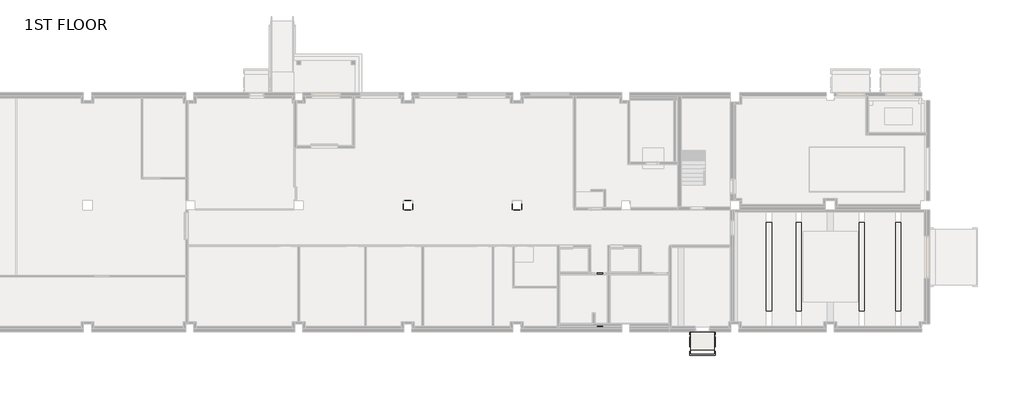
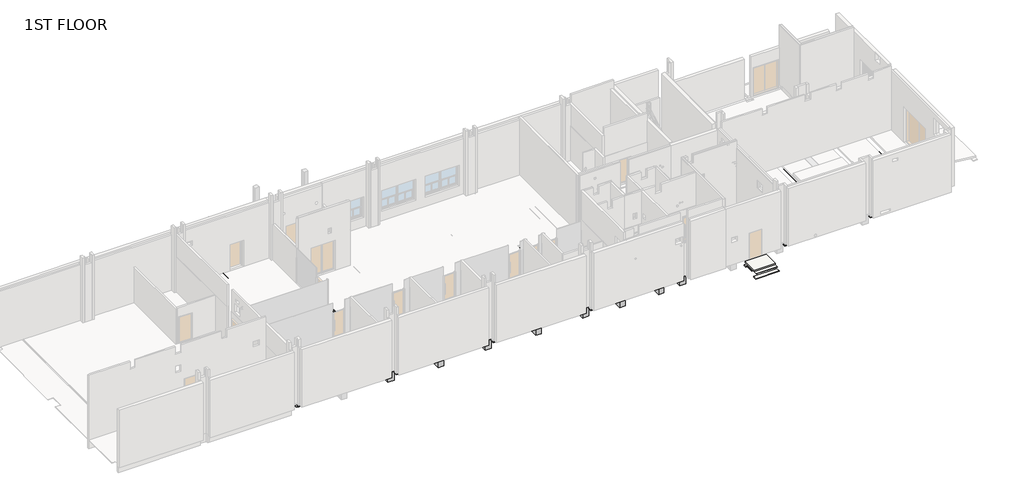
# One storey, part 9 of 15: 19 beams, 7 slabs.
"""IFC4 building model written with IfcOpenShell, lengths in millimetres."""

from ifc_helpers import new_model, si_unit, frame, origin, place, context, project, spatial, polyline, outline, extrude, faceted_brep, element, save

model = new_model("IFC4")

# Units and contexts
model_context = context("Model", 3, world=origin())
ifc_project = project(units=[si_unit("LENGTHUNIT", "METRE", prefix="MILLI")], contexts=[model_context])

# Site, building, storey
site = spatial("IfcSite", under=ifc_project)
building = spatial("IfcBuilding", under=site)
storey = spatial("IfcBuildingStorey", under=building, Name="1ST FLOOR", Elevation=4800.0)

# Beams
placement = place(None, origin())
element("IfcBeam", 1, ObjectType="RC Beam_Rectangular : H_SB_AR S16_TG-UG_500x800_1G2", at=placement, inside=storey, context=model_context, shape_type="Brep", body=[
    faceted_brep([(22650.0, -8350.0, 4800.0), (22650.0, -7850.0, 4800.0), (19225.0, -7850.0, 4800.0), (18775.0, -7850.0, 4800.0), (15400.0000001, -7850.0, 4800.0), (15400.0000001, -8350.0, 4800.0), (18775.0, -8350.0, 4800.0), (19225.0, -8350.0, 4800.0), (22650.0, -7850.0, 4000.0), (19225.0, -7850.0, 4000.0), (18775.0, -7850.0, 4000.0), (15400.0000001, -7850.0, 4000.0), (15400.0000001, -7850.0, 4650.0), (22650.0, -7850.0, 4650.0), (22650.0, -8350.0, 4000.0), (19225.0, -8350.0, 4000.0), (18775.0, -8350.0, 4000.0), (15400.0000001, -8350.0, 4000.0), (22650.0, -8350.0, 4650.0), (15400.0000001, -8350.0, 4650.0)], [[[0, 1, 2, 3, 4, 5, 6, 7]], [[8, 9, 10, 11, 12, 4, 3, 2, 1, 13]], [[11, 10, 9, 8, 14, 15, 16, 17]], [[17, 16, 15, 14, 18, 0, 7, 6, 5, 19]], [[14, 8, 13, 1, 0, 18]], [[5, 4, 12, 11, 17, 19]]]),
])
element("IfcBeam", 2, ObjectType="RC Beam_Rectangular : H_SB_AR S16_TG-UG_500x800_1G2", at=placement, inside=storey, context=model_context, shape_type="Brep", body=[
    faceted_brep([(23350.0, -7850.0, 4800.0), (23350.0, -8350.0, 4800.0), (26775.0, -8350.0, 4800.0), (27225.0, -8350.0, 4800.0), (30650.0, -8350.0, 4800.0), (30650.0, -7850.0, 4800.0), (27225.0, -7850.0, 4800.0), (26775.0, -7850.0, 4800.0), (23350.0, -8350.0, 4000.0), (26775.0, -8350.0, 4000.0), (27225.0, -8350.0, 4000.0), (30650.0, -8350.0, 4000.0), (30650.0, -8350.0, 4650.0), (23350.0, -8350.0, 4650.0), (23350.0, -7850.0, 4000.0), (26775.0, -7850.0, 4000.0), (27225.0, -7850.0, 4000.0), (30650.0, -7850.0, 4000.0), (23350.0, -7850.0, 4650.0), (30650.0, -7850.0, 4650.0)], [[[0, 1, 2, 3, 4, 5, 6, 7]], [[8, 9, 10, 11, 12, 4, 3, 2, 1, 13]], [[11, 10, 9, 8, 14, 15, 16, 17]], [[17, 16, 15, 14, 18, 0, 7, 6, 5, 19]], [[14, 8, 13, 1, 0, 18]], [[5, 4, 12, 11, 17, 19]]]),
])
element("IfcBeam", 3, ObjectType="RC Beam_Rectangular : H_SB_AR S16_TG-UG_500x800_1G2", at=placement, inside=storey, context=model_context, shape_type="Brep", body=[
    faceted_brep([(31350.0, -7850.0, 4800.0), (31350.0, -8350.0, 4800.0), (34775.0, -8350.0, 4800.0), (35225.0, -8350.0, 4800.0), (38650.0, -8350.0, 4800.0), (38650.0, -7850.0, 4800.0), (35225.0, -7850.0, 4800.0), (34775.0, -7850.0, 4800.0), (31350.0, -8350.0, 4000.0), (34775.0, -8350.0, 4000.0), (35225.0, -8350.0, 4000.0), (38650.0, -8350.0, 4000.0), (38650.0, -8350.0, 4650.0), (31350.0, -8350.0, 4650.0), (31350.0, -7850.0, 4000.0), (34775.0, -7850.0, 4000.0), (35225.0, -7850.0, 4000.0), (38650.0, -7850.0, 4000.0), (31350.0, -7850.0, 4650.0), (38650.0, -7850.0, 4650.0)], [[[0, 1, 2, 3, 4, 5, 6, 7]], [[8, 9, 10, 11, 12, 4, 3, 2, 1, 13]], [[11, 10, 9, 8, 14, 15, 16, 17]], [[17, 16, 15, 14, 18, 0, 7, 6, 5, 19]], [[14, 8, 13, 1, 0, 18]], [[5, 4, 12, 11, 17, 19]]]),
])
element("IfcBeam", 4, ObjectType="RC Beam_Rectangular : H_SB_AR S16_TG-UG_500x800_1G2", at=placement, inside=storey, context=model_context, shape_type="Brep", body=[
    faceted_brep([(39350.0, -7850.0, 4800.0), (39350.0, -8350.0, 4800.0), (41675.0, -8350.0, 4800.0), (42125.0, -8350.0, 4800.0), (44875.0, -8350.0, 4800.0), (45325.0, -8350.0, 4800.0), (46650.0, -8350.0, 4800.0), (46650.0, -7850.0, 4800.0), (45325.0, -7850.0, 4800.0), (44875.0, -7850.0, 4800.0), (42125.0, -7850.0, 4800.0), (41675.0, -7850.0, 4800.0), (39350.0, -8350.0, 4000.0), (41675.0, -8350.0, 4000.0), (42125.0, -8350.0, 4000.0), (44875.0, -8350.0, 4000.0), (45325.0, -8350.0, 4000.0), (46650.0, -8350.0, 4000.0), (46650.0, -8350.0, 4650.0), (39350.0, -8350.0, 4650.0), (39350.0, -7850.0, 4000.0), (41675.0, -7850.0, 4000.0), (42125.0, -7850.0, 4000.0), (44875.0, -7850.0, 4000.0), (45325.0, -7850.0, 4000.0), (46650.0, -7850.0, 4000.0), (39350.0, -7850.0, 4650.0), (46650.0, -7850.0, 4650.0)], [[[0, 1, 2, 3, 4, 5, 6, 7, 8, 9, 10, 11]], [[12, 13, 14, 15, 16, 17, 18, 6, 5, 4, 3, 2, 1, 19]], [[17, 16, 15, 14, 13, 12, 20, 21, 22, 23, 24, 25]], [[25, 24, 23, 22, 21, 20, 26, 0, 11, 10, 9, 8, 7, 27]], [[20, 12, 19, 1, 0, 26]], [[7, 6, 18, 17, 25, 27]]]),
])
element("IfcBeam", 5, ObjectType="RC Beam_Rectangular : H_SB_AR S16_TG-UG_500x800_1G1", at=placement, inside=storey, context=model_context, shape_type="Brep", body=[
    faceted_brep([(23200.0, -300.0, 4800.0), (22700.0, -300.0, 4800.0), (22700.0, -7650.0, 4800.0), (23200.0, -7650.0, 4800.0), (23200.0, -7650.0, 4650.0), (23200.0, -7650.0, 4000.0), (23200.0, -300.0, 4000.0), (23200.0, -300.0, 4650.0), (22700.0, -300.0, 4000.0), (22700.0, -7650.0, 4000.0), (22700.0, -300.0, 4650.0), (22700.0, -7650.0, 4650.0)], [[[0, 1, 2, 3]], [[0, 3, 4, 5, 6, 7]], [[8, 6, 5, 9]], [[2, 1, 10, 8, 9, 11]], [[1, 0, 7, 6, 8, 10]], [[3, 2, 11, 9, 5, 4]]]),
])
element("IfcBeam", 6, ObjectType="RC Beam_Rectangular : H_SB_AR S16_TG-UG_450x800_1B1", at=placement, inside=storey, context=model_context, shape_type="Brep", body=[
    faceted_brep([(19225.0, -100.0, 4800.0), (18775.0, -100.0, 4800.0), (18775.0, -7850.0, 4800.0), (19225.0, -7850.0, 4800.0), (19225.0, -7850.0, 4650.0), (19225.0, -7850.0, 4000.0), (19225.0, -100.0, 4000.0), (19225.0, -100.0, 4650.0), (18775.0, -100.0, 4000.0), (18775.0, -7850.0, 4000.0), (18775.0, -100.0, 4650.0), (18775.0, -7850.0, 4650.0)], [[[0, 1, 2, 3]], [[0, 3, 4, 5, 6, 7]], [[8, 6, 5, 9]], [[2, 1, 10, 8, 9, 11]], [[1, 0, 7, 6, 8, 10]], [[3, 2, 11, 9, 5, 4]]]),
])
element("IfcBeam", 7, ObjectType="RC Beam_Rectangular : H_SB_AR S16_TG-UG_500x800_1G1", at=placement, inside=storey, context=model_context, shape_type="Brep", body=[
    faceted_brep([(31250.0, -300.0, 4800.0), (30750.0, -300.0, 4800.0), (30750.0, -7650.0, 4800.0), (31250.0, -7650.0, 4800.0), (31250.0, -7650.0, 4650.0), (31250.0, -7650.0, 4000.0), (31250.0, -300.0, 4000.0), (31250.0, -300.0, 4650.0), (30750.0, -300.0, 4000.0), (30750.0, -7650.0, 4000.0), (30750.0, -300.0, 4650.0), (30750.0, -7650.0, 4650.0)], [[[0, 1, 2, 3]], [[0, 3, 4, 5, 6, 7]], [[8, 6, 5, 9]], [[2, 1, 10, 8, 9, 11]], [[1, 0, 7, 6, 8, 10]], [[3, 2, 11, 9, 5, 4]]]),
])
element("IfcBeam", 8, ObjectType="RC Beam_Rectangular : H_SB_AR S16_TG-UG_450x800_1B1", at=placement, inside=storey, context=model_context, shape_type="Brep", body=[
    faceted_brep([(27225.0, -100.0, 4800.0), (26775.0, -100.0, 4800.0), (26775.0, -7850.0, 4800.0), (27225.0, -7850.0, 4800.0), (27225.0, -7850.0, 4650.0), (27225.0, -7850.0, 4000.0), (27225.0, -100.0, 4000.0), (27225.0, -100.0, 4650.0), (26775.0, -100.0, 4000.0), (26775.0, -7850.0, 4000.0), (26775.0, -100.0, 4650.0), (26775.0, -7850.0, 4650.0)], [[[0, 1, 2, 3]], [[0, 3, 4, 5, 6, 7]], [[8, 6, 5, 9]], [[2, 1, 10, 8, 9, 11]], [[1, 0, 7, 6, 8, 10]], [[3, 2, 11, 9, 5, 4]]]),
])
element("IfcBeam", 9, ObjectType="RC Beam_Rectangular : H_SB_AR S16_TG-UG_450x800_1B1", at=placement, inside=storey, context=model_context, shape_type="Brep", body=[
    faceted_brep([(35225.0, -100.0, 4800.0), (34775.0, -100.0, 4800.0), (34775.0, -7850.0, 4800.0), (35225.0, -7850.0, 4800.0), (35225.0, -7850.0, 4650.0), (35225.0, -7850.0, 4000.0), (35225.0, -100.0, 4000.0), (35225.0, -100.0, 4650.0), (34775.0, -100.0, 4000.0), (34775.0, -7850.0, 4000.0), (34775.0, -100.0, 4650.0), (34775.0, -7850.0, 4650.0)], [[[0, 1, 2, 3]], [[0, 3, 4, 5, 6, 7]], [[8, 6, 5, 9]], [[2, 1, 10, 8, 9, 11]], [[1, 0, 7, 6, 8, 10]], [[3, 2, 11, 9, 5, 4]]]),
])
element("IfcBeam", 10, ObjectType="RC Beam_Rectangular : H_SB_AR S16_TG-UG_500x800_1G1", at=placement, inside=storey, context=model_context, shape_type="Brep", body=[
    faceted_brep([(22750.0, -16700.0, 4800.0), (23250.0, -16700.0, 4800.0), (23250.0, -8350.0, 4800.0), (22750.0, -8350.0, 4800.0), (23250.0, -16700.0, 4650.0), (23250.0, -16700.0, 4000.0), (23250.0, -8350.0, 4000.0), (23250.0, -8350.0, 4650.0), (22750.0, -16700.0, 4000.0), (22750.0, -8350.0, 4000.0), (22750.0, -16700.0, 4650.0), (22750.0, -8350.0, 4650.0)], [[[0, 1, 2, 3]], [[1, 4, 5, 6, 7, 2]], [[5, 8, 9, 6]], [[8, 10, 0, 3, 11, 9]], [[8, 5, 4, 1, 0, 10]], [[3, 2, 7, 6, 9, 11]]]),
])
element("IfcBeam", 11, ObjectType="RC Beam_Rectangular : H_SB_AR S16_TG-UG_500x800_1G1", at=placement, inside=storey, context=model_context, shape_type="Brep", body=[
    faceted_brep([(30750.0, -16700.0, 4800.0), (31250.0, -16700.0, 4800.0), (31250.0, -8350.0, 4800.0), (30750.0, -8350.0, 4800.0), (31250.0, -16700.0, 4650.0), (31250.0, -16700.0, 4000.0), (31250.0, -8350.0, 4000.0), (31250.0, -8350.0, 4650.0), (30750.0, -16700.0, 4000.0), (30750.0, -8350.0, 4000.0), (30750.0, -16700.0, 4650.0), (30750.0, -8350.0, 4650.0)], [[[0, 1, 2, 3]], [[1, 4, 5, 6, 7, 2]], [[5, 8, 9, 6]], [[8, 10, 0, 3, 11, 9]], [[8, 5, 4, 1, 0, 10]], [[3, 2, 7, 6, 9, 11]]]),
])
element("IfcBeam", 12, ObjectType="RC Beam_Rectangular : H_SB_AR S16_TG-UG_500x800_1G1", at=placement, inside=storey, context=model_context, shape_type="Brep", body=[
    faceted_brep([(38750.0000001, -16700.0, 4800.0), (39250.0000001, -16700.0, 4800.0), (39250.0000001, -8350.0, 4800.0), (38750.0000001, -8350.0, 4800.0), (39250.0000001, -16700.0, 4650.0), (39250.0000001, -16700.0, 4000.0), (39250.0000001, -8350.0, 4000.0), (39250.0000001, -8350.0, 4650.0), (38750.0000001, -16700.0, 4000.0), (38750.0000001, -8350.0, 4000.0), (38750.0000001, -16700.0, 4650.0), (38750.0000001, -8350.0, 4650.0)], [[[0, 1, 2, 3]], [[1, 4, 5, 6, 7, 2]], [[5, 8, 9, 6]], [[8, 10, 0, 3, 11, 9]], [[8, 5, 4, 1, 0, 10]], [[3, 2, 7, 6, 9, 11]]]),
])
element("IfcBeam", 13, ObjectType="RC Beam_Rectangular : H_SB_AR S16_TG-UG_450x800_1B1A", at=placement, inside=storey, context=model_context, shape_type="Brep", body=[
    faceted_brep([(26775.0, -16900.0, 4800.0), (27225.0, -16900.0, 4800.0), (27225.0, -8350.0, 4800.0), (26775.0, -8350.0, 4800.0), (27225.0, -16900.0, 4650.0), (27225.0, -16900.0, 4000.0), (27225.0, -8350.0, 4000.0), (27225.0, -8350.0, 4650.0), (26775.0, -16900.0, 4000.0), (26775.0, -8350.0, 4000.0), (26775.0, -8350.0, 4650.0), (26775.0, -16900.0, 4650.0)], [[[0, 1, 2, 3]], [[2, 1, 4, 5, 6, 7]], [[5, 8, 9, 6]], [[0, 3, 10, 9, 8, 11]], [[1, 0, 11, 8, 5, 4]], [[3, 2, 7, 6, 9, 10]]]),
])
element("IfcBeam", 14, ObjectType="RC Beam_Rectangular : H_SB_AR S16_TG-UG_450x800_1B1A", at=placement, inside=storey, context=model_context, shape_type="Brep", body=[
    faceted_brep([(34775.0, -16900.0, 4800.0), (35225.0, -16900.0, 4800.0), (35225.0, -8350.0, 4800.0), (34775.0, -8350.0, 4800.0), (35225.0, -16900.0, 4650.0), (35225.0, -16900.0, 4000.0), (35225.0, -8350.0, 4000.0), (35225.0, -8350.0, 4650.0), (34775.0, -16900.0, 4000.0), (34775.0, -8350.0, 4000.0), (34775.0, -8350.0, 4650.0), (34775.0, -16900.0, 4650.0)], [[[0, 1, 2, 3]], [[2, 1, 4, 5, 6, 7]], [[5, 8, 9, 6]], [[0, 3, 10, 9, 8, 11]], [[1, 0, 11, 8, 5, 4]], [[3, 2, 7, 6, 9, 10]]]),
])
element("IfcBeam", 15, ObjectType="RC Beam_Rectangular : H_SB_AR S16_TG-UG_450x800_1B1A", at=placement, inside=storey, context=model_context, shape_type="Brep", body=[
    faceted_brep([(42125.0, -8350.0, 4800.0), (41675.0, -8350.0, 4800.0), (41675.0, -16900.0, 4800.0), (42125.0, -16900.0, 4800.0), (42125.0, -11075.0, 4800.0), (42125.0, -16900.0, 4700.0), (42125.0, -16900.0, 4550.0), (42125.0, -16900.0, 4000.0), (42125.0, -8350.0, 4000.0), (42125.0, -8350.0, 4650.0), (41675.0, -16900.0, 4000.0), (41675.0, -8350.0, 4000.0), (41675.0, -16900.0, 4650.0), (41675.0, -8350.0, 4650.0)], [[[0, 1, 2, 3, 4]], [[3, 5, 6, 7, 8, 9, 0, 4]], [[7, 10, 11, 8]], [[11, 10, 12, 2, 1, 13]], [[7, 6, 5, 3, 2, 12, 10]], [[1, 0, 9, 8, 11, 13]]]),
])
element("IfcBeam", 16, ObjectType="RC Beam_Rectangular : H_SB_AR S16_TG-UG_450x700_1B1B", at=placement, inside=storey, context=model_context, shape_type="Brep", body=[
    faceted_brep([(44875.0, -13075.0, 4700.0), (45325.0, -13075.0, 4700.0), (45325.0, -13075.0, 4650.0), (45325.0, -13075.0, 4550.0), (45325.0, -13075.0, 4000.0), (44875.0, -13075.0, 4000.0), (44875.0, -13075.0, 4550.0), (44875.0, -13075.0, 4650.0), (44875.0, -16900.0, 4700.0), (45325.0, -16900.0, 4700.0), (45325.0, -16900.0, 4550.0), (45325.0, -16900.0, 4000.0), (44875.0, -16900.0, 4000.0), (44875.0, -16900.0, 4550.0)], [[[0, 1, 2, 3, 4, 5, 6, 7]], [[1, 0, 8, 9]], [[1, 9, 10, 11, 4, 3, 2]], [[5, 4, 11, 12]], [[8, 0, 7, 6, 5, 12, 13]], [[12, 11, 10, 9, 8, 13]]]),
])
element("IfcBeam", 17, ObjectType="RC Beam_Rectangular : H_SB_AR S16_TG-UG_500x700_1G1A", at=placement, inside=storey, context=model_context, shape_type="Brep", body=[
    faceted_brep([(46750.0, -11075.0, 4700.0), (47250.0, -11075.0, 4700.0), (47250.0, -11075.0, 4550.0), (47250.0, -11075.0, 4000.0), (46750.0, -11075.0, 4000.0), (46750.0, -11075.0, 4550.0), (46750.0, -16700.0, 4700.0), (47250.0, -16700.0, 4700.0), (47250.0, -16700.0, 4550.0), (47250.0, -16700.0, 4000.0), (46750.0, -16700.0, 4000.0), (46750.0, -16700.0, 4550.0)], [[[0, 1, 2, 3, 4, 5]], [[1, 0, 6, 7]], [[1, 7, 8, 9, 3, 2]], [[4, 3, 9, 10]], [[6, 0, 5, 4, 10, 11]], [[10, 9, 8, 7, 6, 11]]]),
])
element("IfcBeam", 18, ObjectType="RC Beam_Rectangular : H_SB_AR S16_TG-UG_500x800_1G1A", at=placement, inside=storey, context=model_context, shape_type="Brep", body=[
    faceted_brep([(46750.0, -11075.0, 4000.0), (47250.0, -11075.0, 4000.0), (47250.0, -11075.0, 4650.0), (47250.0, -11075.0, 4700.0), (47250.0, -11075.0, 4800.0), (46750.0, -11075.0, 4800.0), (46750.0, -11075.0, 4700.0), (46750.0, -11075.0, 4650.0), (47249.9999999, -8350.0, 4800.0), (46749.9999999, -8350.0, 4800.0), (47249.9999999, -8350.0, 4000.0), (47249.9999999, -8350.0, 4650.0), (46749.9999999, -8350.0, 4000.0), (46749.9999999, -8350.0, 4650.0)], [[[0, 1, 2, 3, 4, 5, 6, 7]], [[5, 4, 8, 9]], [[2, 1, 10, 11, 8, 4, 3]], [[1, 0, 12, 10]], [[7, 6, 5, 9, 13, 12, 0]], [[9, 8, 11, 10, 12, 13]]]),
])
element("IfcBeam", 19, ObjectType="RC Beam_Rectangular : H_SB_AR S16_TG-UG_450x800_1B1B", at=placement, inside=storey, context=model_context, shape_type="Brep", body=[
    faceted_brep([(44875.0, -13075.0, 4000.0), (45325.0, -13075.0, 4000.0), (45325.0, -13075.0, 4650.0), (45325.0, -13075.0, 4700.0), (45325.0, -13075.0, 4800.0), (44875.0, -13075.0, 4800.0), (44875.0, -13075.0, 4700.0), (44875.0, -13075.0, 4650.0), (45325.0, -8350.0, 4800.0), (44875.0, -8350.0, 4800.0), (45325.0, -8350.0, 4000.0), (45325.0, -8350.0, 4650.0), (44875.0, -8350.0, 4000.0), (44875.0, -8350.0, 4650.0)], [[[0, 1, 2, 3, 4, 5, 6, 7]], [[5, 4, 8, 9]], [[8, 4, 3, 2, 1, 10, 11]], [[1, 0, 12, 10]], [[5, 9, 13, 12, 0, 7, 6]], [[9, 8, 11, 10, 12, 13]]]),
])

# Slabs
element("IfcSlab", 20, ObjectType="H_SF_AR_B08_Stoop_T150", at=placement, inside=storey, context=model_context, shape_type="Brep", body=[
    faceted_brep([(51775.0, -18599.9999926, 4600.0), (51775.0, -18399.9999926, 4600.0), (51775.0, -17662.0, 4600.0), (51775.0, -17312.0, 4600.0), (53475.0, -17312.0, 4600.0), (53475.0, -17662.0, 4600.0), (53475.0, -18399.9999926, 4600.0), (53475.0, -18599.9999926, 4600.0), (51775.0, -18599.9999926, 4750.0), (53475.0, -18599.9999926, 4750.0), (53475.0, -17312.0, 4750.0), (51775.0, -17312.0, 4750.0), (51775.0, -18599.9999926, 4625.0), (53475.0, -18599.9999926, 4625.0)], [[[0, 1, 2, 3, 4, 5, 6, 7]], [[8, 9, 10, 11]], [[3, 2, 1, 0, 12, 8, 11]], [[4, 3, 11, 10]], [[7, 6, 5, 4, 10, 9, 13]], [[0, 7, 13, 9, 8, 12]]]),
])
element("IfcSlab", 21, ObjectType="H_SF_AR_B08_Stoop_T125", at=placement, inside=storey, context=model_context, shape_type="SweptSolid", body=[
    extrude(outline(polyline([(51775.0, -18899.9999926), (51775.0, -18599.9999926), (53475.0, -18599.9999926), (53475.0, -18899.9999926), (51775.0, -18899.9999926)])), frame((0.0, 0.0, 4600.0), z_axis=(0.0, 0.0, 1.0), x_axis=(1.0, 0.0, 0.0)), (0.0, 0.0, 1.0), 25.0),
])
element("IfcSlab", 22, ObjectType="H_SF_AR_S18_Lean_T50", at=placement, inside=storey, context=model_context, shape_type="SweptSolid", body=[
    extrude(outline(polyline([(51675.0, -18999.9999926), (51675.0, -18699.9999926), (53575.0, -18699.9999926), (53575.0, -18999.9999926), (51675.0, -18999.9999926)])), frame((0.0, 0.0, 4250.0), z_axis=(0.0, 0.0, 1.0), x_axis=(1.0, 0.0, 0.0)), (0.0, 0.0, 1.0), 50.0),
])
element("IfcSlab", 23, ObjectType="H_SF_AR_S18_Lean_T50", at=placement, inside=storey, context=model_context, shape_type="SweptSolid", body=[
    extrude(outline(polyline([(51675.0, -17299.9999926), (53575.0, -17299.9999926), (53575.0, -17512.0), (51675.0, -17512.0), (51675.0, -17299.9999926)])), frame((0.0, 0.0, 4400.0), z_axis=(0.0, 0.0, 1.0), x_axis=(1.0, 0.0, 0.0)), (0.0, 0.0, 1.0), 50.0),
])
element("IfcSlab", 24, ObjectType="H_SF_AR_S18_Lean_T50", at=placement, inside=storey, context=model_context, shape_type="Brep", body=[
    faceted_brep([(51675.0, -18399.9999926, 4550.0), (51675.0, -18379.2893145, 4550.0), (51675.0, -17682.7106781, 4550.0), (51675.0, -17662.0, 4550.0), (53575.0, -17662.0, 4550.0), (53575.0, -17682.7106781, 4550.0), (53575.0, -18379.2893145, 4550.0), (53575.0, -18399.9999926, 4550.0), (51675.0, -18399.9999926, 4600.0), (53575.0, -18399.9999926, 4600.0), (53575.0, -17662.0, 4600.0), (51675.0, -17662.0, 4600.0)], [[[0, 1, 2, 3, 4, 5, 6, 7]], [[8, 9, 10, 11]], [[3, 2, 1, 0, 8, 11]], [[4, 3, 11, 10]], [[7, 6, 5, 4, 10, 9]], [[0, 7, 9, 8]]]),
])
element("IfcSlab", 25, ObjectType="H_SF_AR_S18_Lean_T50", at=placement, inside=storey, context=model_context, shape_type="Brep", body=[
    faceted_brep([(19435.0, -1250.0000001, 3840.0), (19435.0, -7640.0, 3840.0), (21750.0000003, -7640.0, 3840.0), (21750.0000003, -8560.0, 3840.0), (19435.0, -8560.0, 3840.0), (19435.0, -15750.0000001, 3840.0), (18565.0, -15750.0000001, 3840.0), (18565.0, -8560.0, 3840.0), (16300.0000001, -8560.0, 3840.0), (16300.0000001, -7640.0, 3840.0), (18565.0, -7640.0, 3840.0), (18565.0, -1250.0000001, 3840.0), (19435.0, -7640.0, 3890.0), (19435.0, -1250.0000001, 3890.0), (18565.0, -1250.0000001, 3890.0), (18565.0, -7640.0, 3890.0), (16300.0000001, -7640.0, 3890.0), (16300.0000001, -8560.0, 3890.0), (18565.0, -8560.0, 3890.0), (18565.0, -15750.0000001, 3890.0), (19435.0, -15750.0000001, 3890.0), (19435.0, -8560.0, 3890.0), (21750.0000003, -8560.0, 3890.0), (21750.0000003, -7640.0, 3890.0)], [[[0, 1, 2, 3, 4, 5, 6, 7, 8, 9, 10, 11]], [[12, 13, 14, 15, 16, 17, 18, 19, 20, 21, 22, 23]], [[1, 0, 13, 12]], [[2, 1, 12, 23]], [[3, 2, 23, 22]], [[4, 3, 22, 21]], [[5, 4, 21, 20]], [[7, 6, 19, 18]], [[8, 7, 18, 17]], [[9, 8, 17, 16]], [[10, 9, 16, 15]], [[11, 10, 15, 14]], [[0, 11, 14, 13]], [[6, 5, 20, 19]]]),
    faceted_brep([(23410.0, -1250.0000001, 3840.0), (23410.0, -6750.0, 3840.0), (22490.0, -6750.0, 3840.0), (22490.0, -1250.0000001, 3840.0), (23410.0, -6750.0, 3890.0), (23410.0, -1250.0000001, 3890.0), (22490.0, -1250.0000001, 3890.0), (22490.0, -6750.0, 3890.0)], [[[0, 1, 2, 3]], [[4, 5, 6, 7]], [[1, 0, 5, 4]], [[2, 1, 4, 7]], [[3, 2, 7, 6]], [[0, 3, 6, 5]]]),
    faceted_brep([(23460.0, -9250.0, 3840.0), (23460.0, -15750.0000001, 3840.0), (22540.0, -15750.0000001, 3840.0), (22540.0, -9250.0, 3840.0), (23460.0, -15750.0000001, 3890.0), (23460.0, -9250.0, 3890.0), (22540.0, -9250.0, 3890.0), (22540.0, -15750.0000001, 3890.0)], [[[0, 1, 2, 3]], [[4, 5, 6, 7]], [[1, 0, 5, 4]], [[2, 1, 4, 7]], [[3, 2, 7, 6]], [[0, 3, 6, 5]]]),
    faceted_brep([(27435.0, -1250.0000001, 3840.0), (27435.0, -7640.0, 3840.0), (29750.0000003, -7640.0, 3840.0), (29750.0000003, -8560.0, 3840.0), (27435.0, -8560.0, 3840.0), (27435.0, -15750.0000001, 3840.0), (26565.0, -15750.0000001, 3840.0), (26565.0, -8560.0, 3840.0), (24249.9999997, -8560.0, 3840.0), (24249.9999997, -7640.0, 3840.0), (26565.0, -7640.0, 3840.0), (26565.0, -1250.0000001, 3840.0), (27435.0, -7640.0, 3890.0), (27435.0, -1250.0000001, 3890.0), (26565.0, -1250.0000001, 3890.0), (26565.0, -7640.0, 3890.0), (24249.9999997, -7640.0, 3890.0), (24249.9999997, -8560.0, 3890.0), (26565.0, -8560.0, 3890.0), (26565.0, -15750.0000001, 3890.0), (27435.0, -15750.0000001, 3890.0), (27435.0, -8560.0, 3890.0), (29750.0000003, -8560.0, 3890.0), (29750.0000003, -7640.0, 3890.0)], [[[0, 1, 2, 3, 4, 5, 6, 7, 8, 9, 10, 11]], [[12, 13, 14, 15, 16, 17, 18, 19, 20, 21, 22, 23]], [[1, 0, 13, 12]], [[2, 1, 12, 23]], [[3, 2, 23, 22]], [[4, 3, 22, 21]], [[5, 4, 21, 20]], [[6, 5, 20, 19]], [[7, 6, 19, 18]], [[8, 7, 18, 17]], [[9, 8, 17, 16]], [[10, 9, 16, 15]], [[11, 10, 15, 14]], [[0, 11, 14, 13]]]),
    faceted_brep([(31459.9999999, -1250.0000001, 3840.0), (31459.9999999, -6750.0, 3840.0), (30539.9999999, -6750.0, 3840.0), (30539.9999999, -1250.0000001, 3840.0), (31459.9999999, -6750.0, 3890.0), (31459.9999999, -1250.0000001, 3890.0), (30539.9999999, -1250.0000001, 3890.0), (30539.9999999, -6750.0, 3890.0)], [[[0, 1, 2, 3]], [[4, 5, 6, 7]], [[1, 0, 5, 4]], [[2, 1, 4, 7]], [[3, 2, 7, 6]], [[0, 3, 6, 5]]]),
    faceted_brep([(31459.9999999, -9250.0, 3840.0), (31459.9999999, -15750.0000001, 3840.0), (30539.9999999, -15750.0000001, 3840.0), (30539.9999999, -9250.0, 3840.0), (31459.9999999, -15750.0000001, 3890.0), (31459.9999999, -9250.0, 3890.0), (30539.9999999, -9250.0, 3890.0), (30539.9999999, -15750.0000001, 3890.0)], [[[0, 1, 2, 3]], [[4, 5, 6, 7]], [[1, 0, 5, 4]], [[2, 1, 4, 7]], [[3, 2, 7, 6]], [[0, 3, 6, 5]]]),
    faceted_brep([(35435.0, -1250.0000001, 3840.0), (35435.0, -7640.0, 3840.0), (37750.0000003, -7640.0, 3840.0), (37750.0000003, -8560.0, 3840.0), (35435.0, -8560.0, 3840.0), (35435.0, -15750.0000001, 3840.0), (34565.0, -15750.0000001, 3840.0), (34565.0, -8560.0, 3840.0), (32250.0000002, -8560.0, 3840.0), (32250.0000002, -7640.0, 3840.0), (34565.0, -7640.0, 3840.0), (34565.0, -1250.0000001, 3840.0), (35435.0, -7640.0, 3890.0), (35435.0, -1250.0000001, 3890.0), (34565.0, -1250.0000001, 3890.0), (34565.0, -7640.0, 3890.0), (32250.0000002, -7640.0, 3890.0), (32250.0000002, -8560.0, 3890.0), (34565.0, -8560.0, 3890.0), (34565.0, -15750.0000001, 3890.0), (35435.0, -15750.0000001, 3890.0), (35435.0, -8560.0, 3890.0), (37750.0000003, -8560.0, 3890.0), (37750.0000003, -7640.0, 3890.0)], [[[0, 1, 2, 3, 4, 5, 6, 7, 8, 9, 10, 11]], [[12, 13, 14, 15, 16, 17, 18, 19, 20, 21, 22, 23]], [[1, 0, 13, 12]], [[2, 1, 12, 23]], [[3, 2, 23, 22]], [[4, 3, 22, 21]], [[5, 4, 21, 20]], [[6, 5, 20, 19]], [[7, 6, 19, 18]], [[8, 7, 18, 17]], [[9, 8, 17, 16]], [[10, 9, 16, 15]], [[11, 10, 15, 14]], [[0, 11, 14, 13]]]),
    faceted_brep([(39459.9999999, -1250.0000001, 3840.0), (39459.9999999, -6750.0, 3840.0), (38539.9999999, -6750.0, 3840.0), (38539.9999999, -1250.0000001, 3840.0), (39459.9999999, -6750.0, 3890.0), (39459.9999999, -1250.0000001, 3890.0), (38539.9999999, -1250.0000001, 3890.0), (38539.9999999, -6750.0, 3890.0)], [[[0, 1, 2, 3]], [[4, 5, 6, 7]], [[1, 0, 5, 4]], [[2, 1, 4, 7]], [[3, 2, 7, 6]], [[0, 3, 6, 5]]]),
    faceted_brep([(39459.9999999, -9250.0, 3840.0), (39459.9999999, -15750.0000001, 3840.0), (38539.9999999, -15750.0000001, 3840.0), (38539.9999999, -9250.0, 3840.0), (39459.9999999, -15750.0000001, 3890.0), (39459.9999999, -9250.0, 3890.0), (38539.9999999, -9250.0, 3890.0), (38539.9999999, -15750.0000001, 3890.0)], [[[0, 1, 2, 3]], [[4, 5, 6, 7]], [[1, 0, 5, 4]], [[2, 1, 4, 7]], [[3, 2, 7, 6]], [[0, 3, 6, 5]]]),
    faceted_brep([(42335.0, -1250.0000001, 3840.0), (42335.0, -7640.0, 3840.0), (44665.0, -7640.0, 3840.0), (44665.0, -1250.0000001, 3840.0), (45535.0, -1250.0000001, 3840.0), (45535.0, -7640.0, 3840.0), (45749.9999999, -7640.0, 3840.0), (45749.9999999, -8560.0, 3840.0), (45535.0, -8560.0, 3840.0), (45535.0, -15750.0000001, 3840.0), (44665.0, -15750.0000001, 3840.0), (44665.0, -8560.0, 3840.0), (42335.0, -8560.0, 3840.0), (42335.0, -15750.0000001, 3840.0), (41465.0, -15750.0000001, 3840.0), (41465.0, -8560.0, 3840.0), (40250.0000001, -8560.0, 3840.0), (40250.0000001, -7640.0, 3840.0), (41465.0, -7640.0, 3840.0), (41465.0, -1250.0000001, 3840.0), (42335.0, -7640.0, 3890.0), (42335.0, -1250.0000001, 3890.0), (41465.0, -1250.0000001, 3890.0), (41465.0, -7640.0, 3890.0), (40250.0000001, -7640.0, 3890.0), (40250.0000001, -8560.0, 3890.0), (41465.0, -8560.0, 3890.0), (41465.0, -15750.0000001, 3890.0), (42335.0, -15750.0000001, 3890.0), (42335.0, -8560.0, 3890.0), (44665.0, -8560.0, 3890.0), (44665.0, -15750.0000001, 3890.0), (45535.0, -15750.0000001, 3890.0), (45535.0, -8560.0, 3890.0), (45749.9999999, -8560.0, 3890.0), (45749.9999999, -7640.0, 3890.0), (45535.0, -7640.0, 3890.0), (45535.0, -1250.0000001, 3890.0), (44665.0, -1250.0000001, 3890.0), (44665.0, -7640.0, 3890.0)], [[[0, 1, 2, 3, 4, 5, 6, 7, 8, 9, 10, 11, 12, 13, 14, 15, 16, 17, 18, 19]], [[20, 21, 22, 23, 24, 25, 26, 27, 28, 29, 30, 31, 32, 33, 34, 35, 36, 37, 38, 39]], [[1, 0, 21, 20]], [[2, 1, 20, 39]], [[3, 2, 39, 38]], [[4, 3, 38, 37]], [[5, 4, 37, 36]], [[6, 5, 36, 35]], [[7, 6, 35, 34]], [[8, 7, 34, 33]], [[9, 8, 33, 32]], [[10, 9, 32, 31]], [[11, 10, 31, 30]], [[12, 11, 30, 29]], [[13, 12, 29, 28]], [[14, 13, 28, 27]], [[15, 14, 27, 26]], [[16, 15, 26, 25]], [[17, 16, 25, 24]], [[18, 17, 24, 23]], [[19, 18, 23, 22]], [[0, 19, 22, 21]]]),
    faceted_brep([(47509.9999996, -1250.0000001, 3840.0), (47509.9999996, -6750.0, 3840.0), (46589.9999996, -6750.0, 3840.0), (46589.9999996, -1250.0000001, 3840.0), (47509.9999996, -6750.0, 3890.0), (47509.9999996, -1250.0000001, 3890.0), (46589.9999996, -1250.0000001, 3890.0), (46589.9999996, -6750.0, 3890.0)], [[[0, 1, 2, 3]], [[4, 5, 6, 7]], [[1, 0, 5, 4]], [[2, 1, 4, 7]], [[3, 2, 7, 6]], [[0, 3, 6, 5]]]),
    faceted_brep([(47459.9999996, -9250.0, 3840.0), (47459.9999996, -15750.0000001, 3840.0), (47300.0, -15750.0000001, 3840.0), (46539.9999996, -15750.0000001, 3840.0), (46539.9999996, -9250.0, 3840.0), (47459.9999996, -15750.0000001, 3890.0), (47459.9999996, -9250.0, 3890.0), (46539.9999996, -9250.0, 3890.0), (46539.9999996, -15750.0000001, 3890.0), (47300.0, -15750.0000001, 3890.0)], [[[0, 1, 2, 3, 4]], [[5, 6, 7, 8, 9]], [[1, 0, 6, 5]], [[1, 5, 9, 8, 3, 2]], [[4, 3, 8, 7]], [[0, 4, 7, 6]]]),
    faceted_brep([(49700.0000002, -8560.0, 3840.0), (48249.9999999, -8560.0, 3840.0), (48249.9999999, -7640.0, 3840.0), (49700.0000002, -7640.0, 3840.0), (48249.9999999, -8560.0, 3890.0), (49700.0000002, -8560.0, 3890.0), (49700.0000002, -7640.0, 3890.0), (48249.9999999, -7640.0, 3890.0)], [[[0, 1, 2, 3]], [[4, 5, 6, 7]], [[1, 0, 5, 4]], [[2, 1, 4, 7]], [[3, 2, 7, 6]], [[0, 3, 6, 5]]]),
    faceted_brep([(50615.0, -15750.0000001, 3840.0), (50615.0, -9250.0, 3840.0), (51485.0, -9250.0, 3840.0), (51485.0, -15750.0000001, 3840.0), (50825.0, -15750.0000001, 3840.0), (50615.0, -9250.0, 3890.0), (50615.0, -15750.0000001, 3890.0), (50825.0, -15750.0000001, 3890.0), (51485.0, -15750.0000001, 3890.0), (51485.0, -9250.0, 3890.0)], [[[0, 1, 2, 3, 4]], [[5, 6, 7, 8, 9]], [[1, 0, 6, 5]], [[2, 1, 5, 9]], [[3, 2, 9, 8]], [[3, 8, 7, 6, 0, 4]]]),
    faceted_brep([(54490.0, -15750.0000001, 3840.0), (54490.0, -9250.0, 3840.0), (55410.0, -9250.0, 3840.0), (55410.0, -15750.0000001, 3840.0), (54490.0, -9250.0, 3890.0), (54490.0, -15750.0000001, 3890.0), (55410.0, -15750.0000001, 3890.0), (55410.0, -9250.0, 3890.0)], [[[0, 1, 2, 3]], [[4, 5, 6, 7]], [[1, 0, 5, 4]], [[2, 1, 4, 7]], [[3, 2, 7, 6]], [[0, 3, 6, 5]]]),
    faceted_brep([(57065.0, -15750.0000001, 3840.0), (57065.0, -9250.0, 3840.0), (57935.0, -9250.0, 3840.0), (57935.0, -15750.0000001, 3840.0), (57065.0, -9250.0, 3890.0), (57065.0, -15750.0000001, 3890.0), (57935.0, -15750.0000001, 3890.0), (57935.0, -9250.0, 3890.0)], [[[0, 1, 2, 3]], [[4, 5, 6, 7]], [[1, 0, 5, 4]], [[2, 1, 4, 7]], [[3, 2, 7, 6]], [[0, 3, 6, 5]]]),
    faceted_brep([(59265.0, -15750.0000001, 3840.0), (59265.0, -9250.0, 3840.0), (60135.0, -9250.0, 3840.0), (60135.0, -15750.0000001, 3840.0), (59265.0, -9250.0, 3890.0), (59265.0, -15750.0000001, 3890.0), (60135.0, -15750.0000001, 3890.0), (60135.0, -9250.0, 3890.0)], [[[0, 1, 2, 3]], [[4, 5, 6, 7]], [[1, 0, 5, 4]], [[2, 1, 4, 7]], [[3, 2, 7, 6]], [[0, 3, 6, 5]]]),
    faceted_brep([(61540.0, -15750.0000001, 3840.0), (61540.0, -9250.0, 3840.0), (62460.0, -9250.0, 3840.0), (62460.0, -15750.0000001, 3840.0), (61540.0, -9250.0, 3890.0), (61540.0, -15750.0000001, 3890.0), (62460.0, -15750.0000001, 3890.0), (62460.0, -9250.0, 3890.0)], [[[0, 1, 2, 3]], [[4, 5, 6, 7]], [[1, 0, 5, 4]], [[2, 1, 4, 7]], [[3, 2, 7, 6]], [[0, 3, 6, 5]]]),
    faceted_brep([(63865.0, -15750.0000001, 3840.0), (63865.0, -9250.0, 3840.0), (64735.0, -9250.0, 3840.0), (64735.0, -15750.0000001, 3840.0), (63865.0, -9250.0, 3890.0), (63865.0, -15750.0000001, 3890.0), (64735.0, -15750.0000001, 3890.0), (64735.0, -9250.0, 3890.0)], [[[0, 1, 2, 3]], [[4, 5, 6, 7]], [[1, 0, 5, 4]], [[2, 1, 4, 7]], [[3, 2, 7, 6]], [[0, 3, 6, 5]]]),
    faceted_brep([(66565.0, -15750.0000001, 3840.0), (66565.0, -9250.0, 3840.0), (67435.0, -9250.0, 3840.0), (67435.0, -15750.0000001, 3840.0), (66565.0, -9250.0, 3890.0), (66565.0, -15750.0000001, 3890.0), (67435.0, -15750.0000001, 3890.0), (67435.0, -9250.0, 3890.0)], [[[0, 1, 2, 3]], [[4, 5, 6, 7]], [[1, 0, 5, 4]], [[2, 1, 4, 7]], [[3, 2, 7, 6]], [[0, 3, 6, 5]]]),
])
element("IfcSlab", 26, ObjectType="H_SF_AR_S18_Lean_T50", at=placement, inside=storey, context=model_context, shape_type="Brep", body=[
    faceted_brep([(15210.0, -8460.0, 4490.0), (18665.0, -8460.0, 4490.0), (18665.0, -16790.0, 4490.0), (15300.0, -16790.0, 4490.0), (15300.0, -16700.0, 4490.0), (15210.0, -16700.0, 4490.0), (18665.0, -8460.0, 4540.0), (15210.0, -8460.0, 4540.0), (15210.0, -16700.0, 4540.0), (15300.0, -16700.0, 4540.0), (15300.0, -16790.0, 4540.0), (18665.0, -16790.0, 4540.0)], [[[0, 1, 2, 3, 4, 5]], [[6, 7, 8, 9, 10, 11]], [[1, 0, 7, 6]], [[2, 1, 6, 11]], [[3, 2, 11, 10]], [[4, 3, 10, 9]], [[5, 4, 9, 8]], [[0, 5, 8, 7]]]),
    faceted_brep([(15400.0000001, -7740.0, 4490.0), (15400.0000001, -7650.0, 4490.0), (15210.0, -7650.0, 4490.0), (15210.0, -300.0, 4490.0), (15300.0, -300.0, 4490.0), (15300.0, -210.0, 4490.0), (18665.0, -210.0, 4490.0), (18665.0, -7740.0, 4490.0), (15400.0000001, -7650.0, 4540.0), (15400.0000001, -7740.0, 4540.0), (18665.0, -7740.0, 4540.0), (18665.0, -210.0, 4540.0), (15300.0, -210.0, 4540.0), (15300.0, -300.0, 4540.0), (15210.0, -300.0, 4540.0), (15210.0, -7650.0, 4540.0)], [[[0, 1, 2, 3, 4, 5, 6, 7]], [[8, 9, 10, 11, 12, 13, 14, 15]], [[1, 0, 9, 8]], [[2, 1, 8, 15]], [[3, 2, 15, 14]], [[4, 3, 14, 13]], [[5, 4, 13, 12]], [[6, 5, 12, 11]], [[7, 6, 11, 10]], [[0, 7, 10, 9]]]),
    faceted_brep([(22640.0, -8460.0, 4490.0), (22640.0, -16790.0, 4490.0), (19335.0, -16790.0, 4490.0), (19335.0, -8460.0, 4490.0), (22640.0, -16790.0, 4540.0), (22640.0, -8460.0, 4540.0), (19335.0, -8460.0, 4540.0), (19335.0, -16790.0, 4540.0)], [[[0, 1, 2, 3]], [[4, 5, 6, 7]], [[1, 0, 5, 4]], [[2, 1, 4, 7]], [[3, 2, 7, 6]], [[0, 3, 6, 5]]]),
    faceted_brep([(22650.0000003, -7740.0, 4490.0), (19335.0, -7740.0, 4490.0), (19335.0, -210.0, 4490.0), (22590.0, -210.0, 4490.0), (22590.0, -7650.0, 4490.0), (22650.0000003, -7650.0, 4490.0), (19335.0, -7740.0, 4540.0), (22650.0000003, -7740.0, 4540.0), (22650.0000003, -7650.0, 4540.0), (22590.0, -7650.0, 4540.0), (22590.0, -210.0, 4540.0), (19335.0, -210.0, 4540.0)], [[[0, 1, 2, 3, 4, 5]], [[6, 7, 8, 9, 10, 11]], [[1, 0, 7, 6]], [[2, 1, 6, 11]], [[3, 2, 11, 10]], [[4, 3, 10, 9]], [[5, 4, 9, 8]], [[0, 5, 8, 7]]]),
    faceted_brep([(23360.0, -8460.0, 4490.0), (26665.0, -8460.0, 4490.0), (26665.0, -16790.0, 4490.0), (23360.0, -16790.0, 4490.0), (26665.0, -8460.0, 4540.0), (23360.0, -8460.0, 4540.0), (23360.0, -16790.0, 4540.0), (26665.0, -16790.0, 4540.0)], [[[0, 1, 2, 3]], [[4, 5, 6, 7]], [[1, 0, 5, 4]], [[2, 1, 4, 7]], [[3, 2, 7, 6]], [[0, 3, 6, 5]]]),
    faceted_brep([(23350.0000003, -7740.0, 4490.0), (23350.0000003, -7650.0, 4490.0), (23310.0, -7650.0, 4490.0), (23310.0, -210.0, 4490.0), (26665.0, -210.0, 4490.0), (26665.0, -7740.0, 4490.0), (23350.0000003, -7650.0, 4540.0), (23350.0000003, -7740.0, 4540.0), (26665.0, -7740.0, 4540.0), (26665.0, -210.0, 4540.0), (23310.0, -210.0, 4540.0), (23310.0, -7650.0, 4540.0)], [[[0, 1, 2, 3, 4, 5]], [[6, 7, 8, 9, 10, 11]], [[1, 0, 7, 6]], [[2, 1, 6, 11]], [[3, 2, 11, 10]], [[4, 3, 10, 9]], [[5, 4, 9, 8]], [[0, 5, 8, 7]]]),
    faceted_brep([(30640.0, -8460.0, 4490.0), (30640.0, -16790.0, 4490.0), (27335.0, -16790.0, 4490.0), (27335.0, -8460.0, 4490.0), (30640.0, -16790.0, 4540.0), (30640.0, -8460.0, 4540.0), (27335.0, -8460.0, 4540.0), (27335.0, -16790.0, 4540.0)], [[[0, 1, 2, 3]], [[4, 5, 6, 7]], [[1, 0, 5, 4]], [[2, 1, 4, 7]], [[3, 2, 7, 6]], [[0, 3, 6, 5]]]),
    faceted_brep([(30650.0000002, -7740.0, 4490.0), (27335.0, -7740.0, 4490.0), (27335.0, -210.0, 4490.0), (30640.0, -210.0, 4490.0), (30640.0, -7650.0, 4490.0), (30650.0000002, -7650.0, 4490.0), (27335.0, -7740.0, 4540.0), (30650.0000002, -7740.0, 4540.0), (30650.0000002, -7650.0, 4540.0), (30640.0, -7650.0, 4540.0), (30640.0, -210.0, 4540.0), (27335.0, -210.0, 4540.0)], [[[0, 1, 2, 3, 4, 5]], [[6, 7, 8, 9, 10, 11]], [[1, 0, 7, 6]], [[2, 1, 6, 11]], [[3, 2, 11, 10]], [[4, 3, 10, 9]], [[5, 4, 9, 8]], [[0, 5, 8, 7]]]),
    faceted_brep([(31360.0, -8460.0, 4490.0), (34665.0, -8460.0, 4490.0), (34665.0, -16790.0, 4490.0), (31360.0, -16790.0, 4490.0), (34665.0, -8460.0, 4540.0), (31360.0, -8460.0, 4540.0), (31360.0, -16790.0, 4540.0), (34665.0, -16790.0, 4540.0)], [[[0, 1, 2, 3]], [[4, 5, 6, 7]], [[1, 0, 5, 4]], [[2, 1, 4, 7]], [[3, 2, 7, 6]], [[0, 3, 6, 5]]]),
    faceted_brep([(31350.0000002, -7740.0, 4490.0), (31350.0000002, -7650.0, 4490.0), (31360.0, -7650.0, 4490.0), (31360.0, -210.0, 4490.0), (34665.0, -210.0, 4490.0), (34665.0, -7740.0, 4490.0), (31350.0000002, -7650.0, 4540.0), (31350.0000002, -7740.0, 4540.0), (34665.0, -7740.0, 4540.0), (34665.0, -210.0, 4540.0), (31360.0, -210.0, 4540.0), (31360.0, -7650.0, 4540.0)], [[[0, 1, 2, 3, 4, 5]], [[6, 7, 8, 9, 10, 11]], [[1, 0, 7, 6]], [[2, 1, 6, 11]], [[3, 2, 11, 10]], [[4, 3, 10, 9]], [[5, 4, 9, 8]], [[0, 5, 8, 7]]]),
    faceted_brep([(38640.0, -8460.0, 4490.0), (38640.0, -16790.0, 4490.0), (35335.0, -16790.0, 4490.0), (35335.0, -8460.0, 4490.0), (38640.0, -16790.0, 4540.0), (38640.0, -8460.0, 4540.0), (35335.0, -8460.0, 4540.0), (35335.0, -16790.0, 4540.0)], [[[0, 1, 2, 3]], [[4, 5, 6, 7]], [[1, 0, 5, 4]], [[2, 1, 4, 7]], [[3, 2, 7, 6]], [[0, 3, 6, 5]]]),
    faceted_brep([(38650.0000001, -7740.0, 4490.0), (35335.0, -7740.0, 4490.0), (35335.0, -210.0, 4490.0), (38640.0, -210.0, 4490.0), (38640.0, -7650.0, 4490.0), (38650.0000001, -7650.0, 4490.0), (35335.0, -7740.0, 4540.0), (38650.0000001, -7740.0, 4540.0), (38650.0000001, -7650.0, 4540.0), (38640.0, -7650.0, 4540.0), (38640.0, -210.0, 4540.0), (35335.0, -210.0, 4540.0)], [[[0, 1, 2, 3, 4, 5]], [[6, 7, 8, 9, 10, 11]], [[1, 0, 7, 6]], [[2, 1, 6, 11]], [[3, 2, 11, 10]], [[4, 3, 10, 9]], [[5, 4, 9, 8]], [[0, 5, 8, 7]]]),
    faceted_brep([(39360.0, -8460.0, 4490.0), (41565.0, -8460.0, 4490.0), (41565.0, -16790.0, 4490.0), (39360.0, -16790.0, 4490.0), (41565.0, -8460.0, 4540.0), (39360.0, -8460.0, 4540.0), (39360.0, -16790.0, 4540.0), (41565.0, -16790.0, 4540.0)], [[[0, 1, 2, 3]], [[4, 5, 6, 7]], [[1, 0, 5, 4]], [[2, 1, 4, 7]], [[3, 2, 7, 6]], [[0, 3, 6, 5]]]),
    faceted_brep([(39350.0000001, -7740.0, 4490.0), (39350.0000001, -7650.0, 4490.0), (39360.0, -7650.0, 4490.0), (39360.0, -210.0, 4490.0), (41565.0, -210.0, 4490.0), (41565.0, -7740.0, 4490.0), (39350.0000001, -7650.0, 4540.0), (39350.0000001, -7740.0, 4540.0), (41565.0, -7740.0, 4540.0), (41565.0, -210.0, 4540.0), (39360.0, -210.0, 4540.0), (39360.0, -7650.0, 4540.0)], [[[0, 1, 2, 3, 4, 5]], [[6, 7, 8, 9, 10, 11]], [[1, 0, 7, 6]], [[2, 1, 6, 11]], [[3, 2, 11, 10]], [[4, 3, 10, 9]], [[5, 4, 9, 8]], [[0, 5, 8, 7]]]),
    faceted_brep([(44765.0, -210.0, 4490.0), (44765.0, -7740.0, 4490.0), (42235.0, -7740.0, 4490.0), (42235.0, -210.0, 4490.0), (44765.0, -7740.0, 4540.0), (44765.0, -210.0, 4540.0), (42235.0, -210.0, 4540.0), (42235.0, -7740.0, 4540.0)], [[[0, 1, 2, 3]], [[4, 5, 6, 7]], [[1, 0, 5, 4]], [[2, 1, 4, 7]], [[3, 2, 7, 6]], [[0, 3, 6, 5]]]),
    faceted_brep([(45435.0, -8460.0, 4490.0), (46640.0, -8460.0, 4490.0), (46640.0, -10654.2893219, 4490.0), (46640.0, -10675.0, 4490.0), (45435.0, -10675.0, 4490.0), (45435.0, -10654.2893219, 4490.0), (45435.0, -8460.0, 4540.0), (45435.0, -10675.0, 4540.0), (46640.0, -10675.0, 4540.0), (46640.0, -8460.0, 4540.0)], [[[0, 1, 2, 3, 4, 5]], [[6, 7, 8, 9]], [[7, 6, 0, 5, 4]], [[1, 0, 6, 9]], [[9, 8, 3, 2, 1]], [[4, 3, 8, 7]]]),
    faceted_brep([(46700.0, -210.0, 4490.0), (46700.0, -300.0, 4490.0), (46690.0, -300.0, 4490.0), (46690.0, -7650.0, 4490.0), (46649.9999999, -7650.0, 4490.0), (46649.9999999, -7740.0, 4490.0), (45435.0, -7740.0, 4490.0), (45435.0, -210.0, 4490.0), (46700.0, -300.0, 4540.0), (46700.0, -210.0, 4540.0), (45435.0, -210.0, 4540.0), (45435.0, -7740.0, 4540.0), (46649.9999999, -7740.0, 4540.0), (46649.9999999, -7650.0, 4540.0), (46690.0, -7650.0, 4540.0), (46690.0, -300.0, 4540.0)], [[[0, 1, 2, 3, 4, 5, 6, 7]], [[8, 9, 10, 11, 12, 13, 14, 15]], [[1, 0, 9, 8]], [[2, 1, 8, 15]], [[3, 2, 15, 14]], [[4, 3, 14, 13]], [[5, 4, 13, 12]], [[6, 5, 12, 11]], [[7, 6, 11, 10]], [[0, 7, 10, 9]]]),
    faceted_brep([(50715.0, -4825.0, 4490.0), (50715.0, -7740.0, 4490.0), (47410.0, -7740.0, 4490.0), (47410.0, -4825.0, 4490.0), (50715.0, -7740.0, 4540.0), (50715.0, -4825.0, 4540.0), (47410.0, -4825.0, 4540.0), (47410.0, -7740.0, 4540.0)], [[[0, 1, 2, 3]], [[4, 5, 6, 7]], [[1, 0, 5, 4]], [[2, 1, 4, 7]], [[3, 2, 7, 6]], [[0, 3, 6, 5]]]),
    faceted_brep([(54590.0, -8460.0, 4490.0), (54590.0, -16790.0, 4490.0), (51385.0, -16790.0, 4490.0), (51385.0, -8460.0, 4490.0), (54590.0, -16790.0, 4540.0), (54590.0, -8460.0, 4540.0), (51385.0, -8460.0, 4540.0), (51385.0, -16790.0, 4540.0)], [[[0, 1, 2, 3]], [[4, 5, 6, 7]], [[1, 0, 5, 4]], [[2, 1, 4, 7]], [[3, 2, 7, 6]], [[0, 3, 6, 5]]]),
    faceted_brep([(57165.0, -16790.0, 4490.0), (55310.0, -16790.0, 4490.0), (55310.0, -8460.0, 4490.0), (57165.0, -8460.0, 4490.0), (55310.0, -16790.0, 4540.0), (57165.0, -16790.0, 4540.0), (57165.0, -8460.0, 4540.0), (55310.0, -8460.0, 4540.0)], [[[0, 1, 2, 3]], [[4, 5, 6, 7]], [[1, 0, 5, 4]], [[2, 1, 4, 7]], [[3, 2, 7, 6]], [[0, 3, 6, 5]]]),
    faceted_brep([(59365.0, -8460.0, 4490.0), (59365.0, -16790.0, 4490.0), (57835.0, -16790.0, 4490.0), (57835.0, -8460.0, 4490.0), (59365.0, -16790.0, 4540.0), (59365.0, -8460.0, 4540.0), (57835.0, -8460.0, 4540.0), (57835.0, -16790.0, 4540.0)], [[[0, 1, 2, 3]], [[4, 5, 6, 7]], [[1, 0, 5, 4]], [[2, 1, 4, 7]], [[3, 2, 7, 6]], [[0, 3, 6, 5]]]),
    faceted_brep([(61640.0, -16790.0, 4490.0), (60035.0, -16790.0, 4490.0), (60035.0, -8460.0, 4490.0), (61640.0, -8460.0, 4490.0), (60035.0, -16790.0, 4540.0), (61640.0, -16790.0, 4540.0), (61640.0, -8460.0, 4540.0), (60035.0, -8460.0, 4540.0)], [[[0, 1, 2, 3]], [[4, 5, 6, 7]], [[1, 0, 5, 4]], [[2, 1, 4, 7]], [[3, 2, 7, 6]], [[0, 3, 6, 5]]]),
    faceted_brep([(63965.0, -8460.0, 4490.0), (63965.0, -16790.0, 4490.0), (62360.0, -16790.0, 4490.0), (62360.0, -8460.0, 4490.0), (63965.0, -16790.0, 4540.0), (63965.0, -8460.0, 4540.0), (62360.0, -8460.0, 4540.0), (62360.0, -16790.0, 4540.0)], [[[0, 1, 2, 3]], [[4, 5, 6, 7]], [[1, 0, 5, 4]], [[2, 1, 4, 7]], [[3, 2, 7, 6]], [[0, 3, 6, 5]]]),
    faceted_brep([(66665.0, -8460.0, 4490.0), (66665.0, -16790.0, 4490.0), (64635.0, -16790.0, 4490.0), (64635.0, -8460.0, 4490.0), (66665.0, -16790.0, 4540.0), (66665.0, -8460.0, 4540.0), (64635.0, -8460.0, 4540.0), (64635.0, -16790.0, 4540.0)], [[[0, 1, 2, 3]], [[4, 5, 6, 7]], [[1, 0, 5, 4]], [[2, 1, 4, 7]], [[3, 2, 7, 6]], [[0, 3, 6, 5]]]),
    faceted_brep([(68700.0, -16790.0, 4490.0), (67335.0, -16790.0, 4490.0), (67335.0, -8460.0, 4490.0), (68790.0, -8460.0, 4490.0), (68790.0, -16700.0, 4490.0), (68700.0, -16700.0, 4490.0), (67335.0, -16790.0, 4540.0), (68700.0, -16790.0, 4540.0), (68700.0, -16700.0, 4540.0), (68790.0, -16700.0, 4540.0), (68790.0, -8460.0, 4540.0), (67335.0, -8460.0, 4540.0)], [[[0, 1, 2, 3, 4, 5]], [[6, 7, 8, 9, 10, 11]], [[1, 0, 7, 6]], [[2, 1, 6, 11]], [[3, 2, 11, 10]], [[4, 3, 10, 9]], [[5, 4, 9, 8]], [[0, 5, 8, 7]]]),
    faceted_brep([(50575.0, -16790.0, 4490.0), (50575.0, -12675.0, 4490.0), (48375.0, -12675.0, 4490.0), (48375.0, -10675.0, 4490.0), (47360.0, -10675.0, 4490.0), (47360.0, -10654.2893219, 4490.0), (47360.0, -8460.0, 4490.0), (50715.0, -8460.0, 4490.0), (50715.0, -16790.0, 4490.0), (50595.7106781, -16790.0, 4490.0), (50575.0, -12675.0, 4540.0), (50575.0, -16790.0, 4540.0), (50715.0, -16790.0, 4540.0), (50715.0, -8460.0, 4540.0), (47360.0, -8460.0, 4540.0), (47360.0, -10675.0, 4540.0), (48375.0, -10675.0, 4540.0), (48375.0, -12675.0, 4540.0)], [[[0, 1, 2, 3, 4, 5, 6, 7, 8, 9]], [[10, 11, 12, 13, 14, 15, 16, 17]], [[1, 0, 11, 10]], [[2, 1, 10, 17]], [[3, 2, 17, 16]], [[4, 3, 16, 15]], [[15, 14, 6, 5, 4]], [[7, 6, 14, 13]], [[8, 7, 13, 12]], [[12, 11, 0, 9, 8]]]),
    faceted_brep([(44765.0, -12675.0, 4490.0), (44675.0, -12675.0, 4490.0), (44675.0, -10675.0, 4490.0), (42235.0, -10675.0, 4490.0), (42235.0, -10654.2893219, 4490.0), (42235.0, -8460.0, 4490.0), (44765.0, -8460.0, 4490.0), (44765.0, -12654.2893219, 4490.0), (44765.0, -12675.0, 4540.0), (44765.0, -8460.0, 4540.0), (42235.0, -8460.0, 4540.0), (42235.0, -10675.0, 4540.0), (44675.0, -10675.0, 4540.0), (44675.0, -12675.0, 4540.0)], [[[0, 1, 2, 3, 4, 5, 6, 7]], [[8, 9, 10, 11, 12, 13]], [[9, 8, 0, 7, 6]], [[1, 0, 8, 13]], [[2, 1, 13, 12]], [[3, 2, 12, 11]], [[11, 10, 5, 4, 3]], [[6, 5, 10, 9]]]),
])

save(model, "model.ifc")

# Revit data of these elements
# Type "RC Beam_Rectangular : H_SB_AR S16_TG-UG_500x800_1G2"
#   Type Comments = "CV-UG"
#   중앙부 하부근 = ""
#   중앙부 상부근 = ""
#   중앙부 보조근 = ""
#   중앙부 늑근 = ""
#   외단부 하부근 = ""
#   외단부 상부근 = ""
#   외단부 보조근 = ""
#   외단부 늑근 = ""
#   부호 = "TG3"
#   내단부 하부근 = ""
#   내단부 상부근 = ""
#   내단부 보조근 = ""
#   내단부 늑근 = ""
#   ALL 하부근 = "3-D20"
#   ALL 상부근 = "3-D20"
#   ALL 보조근 = ""
#   ALL 늑근 = "2-D10 @120"
#   H_Rebar Ratio = 0.14
#   Width = 500 mm
#   Height = 800 mm
#   Length [instance default] = 1524 mm
#   b = 500 mm
#   h = 800 mm
#   hec_material3 [instance default] = none
#   hec_material2 [instance default] = none
#   hec_material1 [instance default] = none
#   Structural Material [instance default] = none
#   Assembly Code = ""
# Type "RC Beam_Rectangular : H_SB_AR S16_TG-UG_500x800_1G1"
#   Type Comments = "CV-UG"
#   중앙부 하부근 = ""
#   중앙부 상부근 = ""
#   중앙부 보조근 = ""
#   중앙부 늑근 = ""
#   외단부 하부근 = ""
#   외단부 상부근 = ""
#   외단부 보조근 = ""
#   외단부 늑근 = ""
#   부호 = "TG3"
#   내단부 하부근 = ""
#   내단부 상부근 = ""
#   내단부 보조근 = ""
#   내단부 늑근 = ""
#   ALL 하부근 = "3-D20"
#   ALL 상부근 = "3-D20"
#   ALL 보조근 = ""
#   ALL 늑근 = "2-D10 @120"
#   H_Rebar Ratio = 0.14
#   Width = 500 mm
#   Height = 800 mm
#   Length [instance default] = 1524 mm
#   b = 500 mm
#   h = 800 mm
#   hec_material3 [instance default] = none
#   hec_material2 [instance default] = none
#   hec_material1 [instance default] = none
#   Structural Material [instance default] = none
#   Assembly Code = ""
# Type "RC Beam_Rectangular : H_SB_AR S16_TG-UG_450x800_1B1"
#   Type Comments = "CV-UG"
#   중앙부 하부근 = ""
#   중앙부 상부근 = ""
#   중앙부 보조근 = ""
#   중앙부 늑근 = ""
#   외단부 하부근 = ""
#   외단부 상부근 = ""
#   외단부 보조근 = ""
#   외단부 늑근 = ""
#   부호 = "TG3"
#   내단부 하부근 = ""
#   내단부 상부근 = ""
#   내단부 보조근 = ""
#   내단부 늑근 = ""
#   ALL 하부근 = "3-D20"
#   ALL 상부근 = "3-D20"
#   ALL 보조근 = ""
#   ALL 늑근 = "2-D10 @120"
#   H_Rebar Ratio = 0.14
#   Width = 450 mm
#   Height = 800 mm
#   Length [instance default] = 1524 mm
#   b = 450 mm
#   h = 800 mm
#   hec_material3 [instance default] = none
#   hec_material2 [instance default] = none
#   hec_material1 [instance default] = none
#   Structural Material [instance default] = none
#   Assembly Code = ""
# Type "RC Beam_Rectangular : H_SB_AR S16_TG-UG_450x800_1B1A"
#   Type Comments = "CV-UG"
#   중앙부 하부근 = ""
#   중앙부 상부근 = ""
#   중앙부 보조근 = ""
#   중앙부 늑근 = ""
#   외단부 하부근 = ""
#   외단부 상부근 = ""
#   외단부 보조근 = ""
#   외단부 늑근 = ""
#   부호 = "TG3"
#   내단부 하부근 = ""
#   내단부 상부근 = ""
#   내단부 보조근 = ""
#   내단부 늑근 = ""
#   ALL 하부근 = "3-D20"
#   ALL 상부근 = "3-D20"
#   ALL 보조근 = ""
#   ALL 늑근 = "2-D10 @120"
#   H_Rebar Ratio = 0.14
#   Width = 450 mm
#   Height = 800 mm
#   Length [instance default] = 1524 mm
#   b = 450 mm
#   h = 800 mm
#   hec_material3 [instance default] = none
#   hec_material2 [instance default] = none
#   hec_material1 [instance default] = none
#   Structural Material [instance default] = none
#   Assembly Code = ""
# Type "RC Beam_Rectangular : H_SB_AR S16_TG-UG_450x700_1B1B"
#   Type Comments = "CV-UG"
#   중앙부 하부근 = ""
#   중앙부 상부근 = ""
#   중앙부 보조근 = ""
#   중앙부 늑근 = ""
#   외단부 하부근 = ""
#   외단부 상부근 = ""
#   외단부 보조근 = ""
#   외단부 늑근 = ""
#   부호 = "TG3"
#   내단부 하부근 = ""
#   내단부 상부근 = ""
#   내단부 보조근 = ""
#   내단부 늑근 = ""
#   ALL 하부근 = "3-D20"
#   ALL 상부근 = "3-D20"
#   ALL 보조근 = ""
#   ALL 늑근 = "2-D10 @120"
#   H_Rebar Ratio = 0.14
#   Width = 450 mm
#   Height = 700 mm
#   Length [instance default] = 1524 mm
#   b = 450 mm
#   h = 700 mm
#   hec_material3 [instance default] = none
#   hec_material2 [instance default] = none
#   hec_material1 [instance default] = none
#   Structural Material [instance default] = none
#   Assembly Code = ""
# Type "RC Beam_Rectangular : H_SB_AR S16_TG-UG_500x700_1G1A"
#   Type Comments = "CV-UG"
#   중앙부 하부근 = ""
#   중앙부 상부근 = ""
#   중앙부 보조근 = ""
#   중앙부 늑근 = ""
#   외단부 하부근 = ""
#   외단부 상부근 = ""
#   외단부 보조근 = ""
#   외단부 늑근 = ""
#   부호 = "TG3"
#   내단부 하부근 = ""
#   내단부 상부근 = ""
#   내단부 보조근 = ""
#   내단부 늑근 = ""
#   ALL 하부근 = "3-D20"
#   ALL 상부근 = "3-D20"
#   ALL 보조근 = ""
#   ALL 늑근 = "2-D10 @120"
#   H_Rebar Ratio = 0.14
#   Width = 500 mm
#   Height = 700 mm
#   Length [instance default] = 1524 mm
#   b = 500 mm
#   h = 700 mm
#   hec_material3 [instance default] = none
#   hec_material2 [instance default] = none
#   hec_material1 [instance default] = none
#   Structural Material [instance default] = none
#   Assembly Code = ""
# Type "RC Beam_Rectangular : H_SB_AR S16_TG-UG_500x800_1G1A"
#   Type Comments = "CV-UG"
#   중앙부 하부근 = ""
#   중앙부 상부근 = ""
#   중앙부 보조근 = ""
#   중앙부 늑근 = ""
#   외단부 하부근 = ""
#   외단부 상부근 = ""
#   외단부 보조근 = ""
#   외단부 늑근 = ""
#   부호 = "TG3"
#   내단부 하부근 = ""
#   내단부 상부근 = ""
#   내단부 보조근 = ""
#   내단부 늑근 = ""
#   ALL 하부근 = "3-D20"
#   ALL 상부근 = "3-D20"
#   ALL 보조근 = ""
#   ALL 늑근 = "2-D10 @120"
#   H_Rebar Ratio = 0.14
#   Width = 500 mm
#   Height = 800 mm
#   Length [instance default] = 1524 mm
#   b = 500 mm
#   h = 800 mm
#   hec_material3 [instance default] = none
#   hec_material2 [instance default] = none
#   hec_material1 [instance default] = none
#   Structural Material [instance default] = none
#   Assembly Code = ""
# Type "RC Beam_Rectangular : H_SB_AR S16_TG-UG_450x800_1B1B"
#   Type Comments = "CV-UG"
#   중앙부 하부근 = ""
#   중앙부 상부근 = ""
